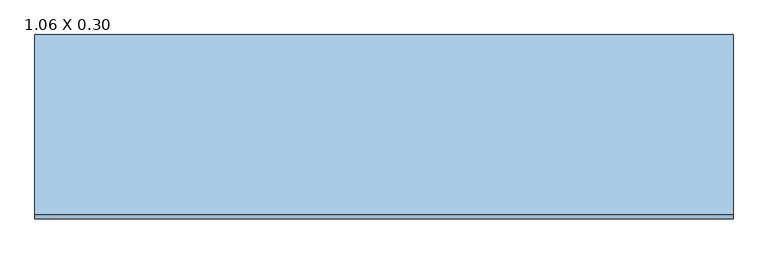
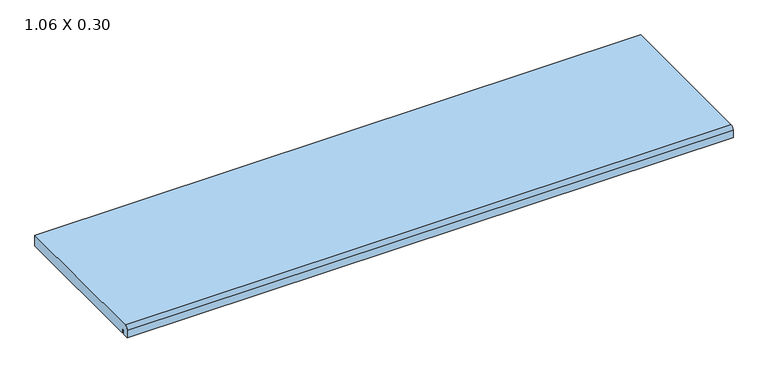
"""IFC4 building model written with IfcOpenShell, lengths in millimetres: window geometry, .CC_ND 300_PEDRA_PEITORIL RETO : 1.06 X 0.30."""

import ifcopenshell
import ifcopenshell.guid

model = None  # the IFC model being written
_history = None  # IfcOwnerHistory: only IFC2X3 demands one
_inside = {}  # id of a spatial element -> (the spatial element, [elements in it])
_under = {}  # id of a project, library or spatial element -> (it, [spatial elements below it])
_declared = {}  # id of a project -> (the project, [libraries it declares])
_typed = {}  # id of a type object -> (the type object, [elements of that type])
_made_of = {}  # id of a material, layer set ... -> (it, [elements and type objects made of it])


def new_model(schema):
    """Start an empty IFC model of exactly this schema.

    Asked for "IFC4X3", IfcOpenShell would pick the latest addendum, in which some entities
    have other attributes; the version numbers below select the first issue.
    IFC2X3 requires an IfcOwnerHistory on every rooted entity: one is made here for all.
    """
    global model, _history
    if schema == "IFC4X3":
        model = ifcopenshell.file(schema_version=(4, 3, 0, 0))
    else:
        model = ifcopenshell.file(schema=schema)
    _inside.clear()
    _under.clear()
    _declared.clear()
    _typed.clear()
    _made_of.clear()
    _history = None
    if model.schema == "IFC2X3":
        org = make("IfcOrganization", Name="unknown")
        user = make(
            "IfcPersonAndOrganization",
            ThePerson=make("IfcPerson", FamilyName="unknown"),
            TheOrganization=org,
        )
        app = make(
            "IfcApplication",
            ApplicationDeveloper=org,
            Version="unknown",
            ApplicationFullName="unknown",
            ApplicationIdentifier="unknown",
        )
        _history = make(
            "IfcOwnerHistory",
            OwningUser=user,
            OwningApplication=app,
            ChangeAction="ADDED",
            CreationDate=0,
        )
    return model


def make(cls, **values):
    """One entity of the class cls with the attributes given. An attribute that is None is left unset."""
    return model.create_entity(
        cls, **{name: value for name, value in values.items() if value is not None}
    )


def rooted(cls, **values):
    """An entity with a GlobalId (a new one), such as an element, a storey or a relation."""
    return make(cls, GlobalId=ifcopenshell.guid.new(), OwnerHistory=_history, **values)


def si_unit(unit_type, name, prefix=None):
    """IfcSIUnit, for example si_unit("LENGTHUNIT", "METRE", prefix="MILLI")."""
    return make("IfcSIUnit", UnitType=unit_type, Prefix=prefix, Name=name)


def assignment(units):
    """IfcUnitAssignment: the units of a project."""
    return None if units is None else make("IfcUnitAssignment", Units=units)


def point(xyz):
    """IfcCartesianPoint."""
    return None if xyz is None else make("IfcCartesianPoint", Coordinates=xyz)


def direction(xyz):
    """IfcDirection."""
    return None if xyz is None else make("IfcDirection", DirectionRatios=xyz)


def frame(location, z_axis=None, x_axis=None):
    """IfcAxis2Placement3D, a coordinate frame: its origin and axes. An axis left out is left unset."""
    return make(
        "IfcAxis2Placement3D",
        Location=point(location),
        Axis=direction(z_axis),
        RefDirection=direction(x_axis),
    )


def frame_2d(location, x_axis=None):
    """IfcAxis2Placement2D, a coordinate frame in the plane: its origin and x axis."""
    return make(
        "IfcAxis2Placement2D", Location=point(location), RefDirection=direction(x_axis)
    )


def origin():
    """The frame at (0, 0, 0) with its axes left unset."""
    return frame((0.0, 0.0, 0.0))


def place(relative_to, where):
    """IfcLocalPlacement: puts the frame where relative to a parent placement (None: the world)."""
    return make(
        "IfcLocalPlacement", PlacementRelTo=relative_to, RelativePlacement=where
    )


def context(
    kind, dimensions, precision=None, world=None, true_north=None, identifier=None
):
    """IfcGeometricRepresentationContext, for example the 3D "Model" context."""
    return make(
        "IfcGeometricRepresentationContext",
        ContextIdentifier=identifier,
        ContextType=kind,
        CoordinateSpaceDimension=dimensions,
        Precision=precision,
        WorldCoordinateSystem=world,
        TrueNorth=true_north,
    )


def project(units=None, contexts=None):
    """IfcProject with its units and contexts."""
    return rooted(
        "IfcProject",
        Name="project",
        RepresentationContexts=contexts,
        UnitsInContext=assignment(units),
    )


def spatial(cls, under=None, at=None, **own):
    """A site, building, storey or space (cls), placed at a placement, below another one or the project."""
    s = rooted(cls, ObjectPlacement=at, **own)
    if under is not None:
        _under.setdefault(under.id(), (under, []))[1].append(s)
    return s


def polyline(points):
    """IfcPolyline through the points."""
    return make("IfcPolyline", Points=[point(p) for p in points])


def circle_curve(where, radius):
    """IfcCircle in the frame where."""
    return make("IfcCircle", Position=where, Radius=radius)


def trimmed(basis, trim1, trim2, sense, master):
    """IfcTrimmedCurve: the piece of a basis curve between two trims."""
    return make(
        "IfcTrimmedCurve",
        BasisCurve=basis,
        Trim1=trim1,
        Trim2=trim2,
        SenseAgreement=sense,
        MasterRepresentation=master,
    )


def segment(curve, same_sense, transition):
    """IfcCompositeCurveSegment."""
    return make(
        "IfcCompositeCurveSegment",
        Transition=transition,
        SameSense=same_sense,
        ParentCurve=curve,
    )


def composite_curve(segments, self_intersect=None):
    """IfcCompositeCurve: segments joined end to end."""
    return make("IfcCompositeCurve", Segments=segments, SelfIntersect=self_intersect)


def outline(outer, holes=None, kind="AREA"):
    """IfcArbitraryClosedProfileDef: a profile drawn as a closed curve; with holes, ...WithVoids."""
    if holes is None:
        return make("IfcArbitraryClosedProfileDef", ProfileType=kind, OuterCurve=outer)
    return make(
        "IfcArbitraryProfileDefWithVoids",
        ProfileType=kind,
        OuterCurve=outer,
        InnerCurves=holes,
    )


def extrude(swept, where, along, depth):
    """IfcExtrudedAreaSolid: the profile swept, set in the frame where, extruded along a direction by depth."""
    return make(
        "IfcExtrudedAreaSolid",
        SweptArea=swept,
        Position=where,
        ExtrudedDirection=direction(along),
        Depth=depth,
    )


def shape(context_of_items, identifier, shape_type, items):
    """IfcShapeRepresentation: the items that make up one representation, for example the "Body"."""
    return make(
        "IfcShapeRepresentation",
        ContextOfItems=context_of_items,
        RepresentationIdentifier=identifier,
        RepresentationType=shape_type,
        Items=items,
    )


def source(mapping_origin, context_of_items, identifier, shape_type, items):
    """IfcRepresentationMap: a shape defined once, which mapped items show again and again."""
    return make(
        "IfcRepresentationMap",
        MappingOrigin=mapping_origin,
        MappedRepresentation=shape(context_of_items, identifier, shape_type, items),
    )


def transform(
    local_origin,
    x_axis=None,
    y_axis=None,
    z_axis=None,
    scale=None,
    scale2=None,
    scale3=None,
    uniform=True,
):
    """IfcCartesianTransformationOperator3D, or its non-uniform kind. x_axis, y_axis, z_axis: its Axis1, 2, 3."""
    if uniform:
        return make(
            "IfcCartesianTransformationOperator3D",
            Axis1=direction(x_axis),
            Axis2=direction(y_axis),
            LocalOrigin=point(local_origin),
            Scale=scale,
            Axis3=direction(z_axis),
        )
    return make(
        "IfcCartesianTransformationOperator3DnonUniform",
        Axis1=direction(x_axis),
        Axis2=direction(y_axis),
        LocalOrigin=point(local_origin),
        Scale=scale,
        Axis3=direction(z_axis),
        Scale2=scale2,
        Scale3=scale3,
    )


def mapped(mapping_source, mapping_target):
    """IfcMappedItem: shows the shape of a source again, moved by a transform."""
    return make(
        "IfcMappedItem", MappingSource=mapping_source, MappingTarget=mapping_target
    )


def made_of(thing, what):
    """Note that an element or type object is made of a material, layer set ...; save() writes the relation."""
    if what is not None:
        _made_of.setdefault(what.id(), (what, []))[1].append(thing)
    return thing


def element(
    cls,
    number,
    at=None,
    inside=None,
    cuts=None,
    type_object=None,
    material=None,
    context=None,
    identifier="Body",
    shape_type=None,
    held_by="IfcProductDefinitionShape",
    body=None,
    shapes=None,
    **own,
):
    """One element of the class cls, such as IfcWall. Its Tag is "e" and its number.

    at: its placement. inside: the storey or other place that contains it. cuts: it is an
    opening in that element (IfcRelVoidsElement). A single representation is given by context,
    identifier, shape_type and body (its items); several are given by shapes. held_by: the class
    of the entity that holds the representations. save() writes the other relations.
    """
    e = rooted(cls, Tag="e%d" % number, ObjectPlacement=at, **own)
    if body is not None:
        shapes = [shape(context, identifier, shape_type, body)]
    if shapes is not None:
        e.Representation = make(held_by, Representations=shapes)
    if inside is not None:
        _inside.setdefault(inside.id(), (inside, []))[1].append(e)
    if cuts is not None:
        rooted(
            "IfcRelVoidsElement", RelatingBuildingElement=cuts, RelatedOpeningElement=e
        )
    if type_object is not None:
        _typed.setdefault(type_object.id(), (type_object, []))[1].append(e)
    return made_of(e, material)


def aggregate(whole, parts):
    """IfcRelAggregates: a whole, such as a stair, and the parts it consists of."""
    return rooted("IfcRelAggregates", RelatingObject=whole, RelatedObjects=parts)


def save(model, path):
    """Write the relations noted so far, then the file.

    IfcRelAggregates (storeys below a building ...), IfcRelContainedInSpatialStructure (elements
    in a storey), IfcRelDefinesByType, IfcRelAssociatesMaterial and IfcRelDeclares: one each for
    every whole, place, type object, material and project.
    """
    for whole, parts in _under.values():
        aggregate(whole, parts)
    for where, things in _inside.values():
        rooted(
            "IfcRelContainedInSpatialStructure",
            RelatedElements=things,
            RelatingStructure=where,
        )
    for kind, things in _typed.values():
        rooted("IfcRelDefinesByType", RelatedObjects=things, RelatingType=kind)
    for what, things in _made_of.values():
        rooted("IfcRelAssociatesMaterial", RelatedObjects=things, RelatingMaterial=what)
    for by, libraries in _declared.values():
        rooted("IfcRelDeclares", RelatingContext=by, RelatedDefinitions=libraries)
    model.write(path)


def window_1_06_x_0_30_7e01d648(model_context):
    return source(origin(), model_context, "Body", "SweptSolid", [
        extrude(outline(composite_curve([segment(polyline([(-132.5083081, 1480.0), (-132.5083081, 1488.1993124), (-137.2619526, 1488.1993124), (-137.2619526, 1480.0), (-148.0, 1480.0), (-148.0, 1493.3808343)]), True, "CONTINUOUS"), segment(trimmed(circle_curve(frame_2d((-141.3808343, 1493.3808343)), 6.6191657), [point((-148.0, 1493.3808343))], [point((-141.3808343, 1500.0))], False, "CARTESIAN"), True, "CONTINUOUS"), segment(polyline([(-141.3808343, 1500.0), (132.0, 1500.0), (132.0, 1480.0), (-132.5083081, 1480.0)]), True, "CONTINUOUS")], self_intersect=False)), frame((-530.0, 0.0, 0.0), z_axis=(1.0, 0.0, 0.0), x_axis=(0.0, 1.0, 0.0)), (0.0, 0.0, 1.0), 1060.0),
    ])


if __name__ == "__main__":
    model = new_model("IFC4")
    model_context = context("Model", 3, world=origin())
    ifc_project = project(units=[si_unit("LENGTHUNIT", "METRE", prefix="MILLI")], contexts=[model_context])
    site = spatial("IfcSite", under=ifc_project)
    building = spatial("IfcBuilding", under=site)
    placement = place(None, origin())
    window_1_06_x_0_30_shape = window_1_06_x_0_30_7e01d648(model_context)
    element("IfcWindow", 1, ObjectType=".CC_ND 300_PEDRA_PEITORIL RETO : 1.06 X 0.30", at=placement, inside=building, context=model_context, shape_type="MappedRepresentation", body=[
        mapped(window_1_06_x_0_30_shape, transform((0.0, 0.0, 0.0), x_axis=(1.0, 0.0, 0.0), y_axis=(0.0, 1.0, 0.0), z_axis=(0.0, 0.0, 1.0))),
    ])
    save(model, "model.ifc")

# Revit data of these elements
# Type ".CC_ND 300_PEDRA_PEITORIL RETO : 1.06 X 0.30"
#   Type Mark = "68"
#   Largura da pedra [instance default] = 0.26 m
#   Extensão interior peitoril [instance default] = 0.03 m
#   Extensão exterior peitoril [instance default] = 0.03 m
#   Espessura = 0.02 m
#   Comprimento = 1.06 m
#   Altura-padrão do peitoril = 1.48 m
#   Peitoril = .GRANITO_BRANCO_ITAUNAS
#   Rough Width = 0
#   Rough Height = 0
#   Height = 0
#   Wall Closure = (empty or 0)
#   Width = 0
# Element 1 (IfcWindow, ".CC_ND 300_PEDRA_PEITORIL RETO : 1.06 X 0.30")
#   Largura da pedra = 0.28 m
#   Extensão interior peitoril = 0.014 m
#   Materials on its faces: ".GRANITO_BRANCO_ITAUNAS"
# Materials
#   ".GRANITO_BRANCO_ITAUNAS": class ".CC_PEDRA REVEST.", colour RGB 202 195 174, transparency 0, Description = "Revestimento em granito", Cost = 0
